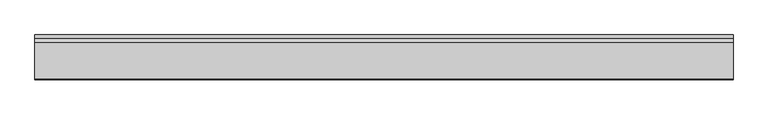
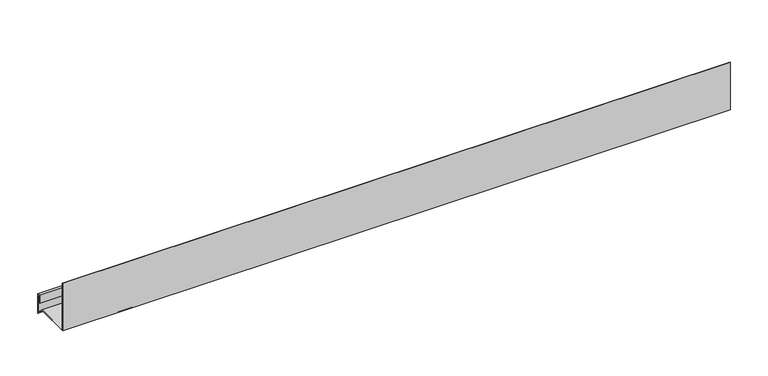
"""IFC4 building model written with IfcOpenShell, lengths in millimetres: proxy geometry, Generic Models 7:Generic Models 1:337419:Generic Models 1:337419 : Generic Models 7:Generic Models 1:337419:2 : Generic Models 7:Generic Models 1:337419:Generic Models 1:337419 : Generic Models 7:Generic Models 1:337419:301336."""

from ifc_helpers import new_model, si_unit, frame, origin, place, context, project, spatial, polyline, outline, extrude, source, transform, mapped, element, save


def generic_models_337c40a0(model_context):
    return source(origin(), model_context, "Body", "SweptSolid", [
        extrude(outline(polyline([(-536494.6078125, 2509.7246799), (-536489.8453125, 2509.7246799), (-536489.8453125, 2477.9746799), (-536501.0706327, 2489.2), (-536554.8784109, 2489.2), (-536554.8784109, 2565.4), (-536554.0846609, 2565.4), (-536554.0846609, 2489.99375), (-536500.7418507, 2489.99375), (-536490.6390625, 2479.8909619), (-536490.6390625, 2508.9309299), (-536493.8140625, 2508.9309299), (-536493.8140625, 2497.0246799), (-536494.6078125, 2497.0246799), (-536494.6078125, 2509.7246799)])), frame((592715.7367242, 0.0, 0.0), z_axis=(1.0, 0.0, 0.0), x_axis=(0.0, 1.0, 0.0)), (0.0, 0.0, 1.0), 1016.0),
    ])


if __name__ == "__main__":
    model = new_model("IFC4")
    model_context = context("Model", 3, world=origin())
    ifc_project = project(units=[si_unit("LENGTHUNIT", "METRE", prefix="MILLI")], contexts=[model_context])
    site = spatial("IfcSite", under=ifc_project)
    building = spatial("IfcBuilding", under=site)
    placement = place(None, origin())
    generic_models_shape = generic_models_337c40a0(model_context)
    element("IfcBuildingElementProxy", 1, Name="Generic Models 7:Generic Models 1:337419:Generic Models 1:337419 : Generic Models 7:Generic Models 1:337419:2 : Generic Models 7:Generic Models 1:337419:Generic Models 1:337419 : Generic Models 7:Generic Models 1:337419:301336", ObjectType="Generic Models 7:Generic Models 1:337419:Generic Models 1:337419 : Generic Models 7:Generic Models 1:337419:2 : Generic Models 7:Generic Models 1:337419:Generic Models 1:337419 : Generic Models 7:Generic Models 1:337419:301336", at=placement, inside=building, context=model_context, shape_type="MappedRepresentation", body=[
        mapped(generic_models_shape, transform((0.0, 0.0, 0.0), x_axis=(1.0, 0.0, 0.0), y_axis=(0.0, 1.0, 0.0), z_axis=(0.0, 0.0, 1.0))),
    ])
    save(model, "model.ifc")

# Revit data of these elements
# Type "Generic Models 7:Generic Models 1:337419:Generic Models 1:337419 : Generic Models 7:Generic Models 1:337419:2 : Generic Models 7:Generic Models 1:337419:Generic Models 1:337419 : Generic Models 7:Generic Models 1:337419:301336"
#   NameOverride = "Generic Models 7:Generic Models 1:337419:Generic Models 1:337419 : Generic Models 7:Generic Models 1:337419:301336"
#   ObjectTypeOverride = "Generic Models 1:337419 : Generic Models 7:Generic Models 1:337419"
#   Reference = "Generic Models 1"
#   Tag = "301336"
# Element 1 (IfcBuildingElementProxy, "Generic Models 7:Generic Models 1:337419:Generic Models 1:337419 : Generic Models 7:Generic Models 1:337419:2 : Generic Models 7:Generic Models 1:337419:Generic Models 1:337419 : Generic Models 7:Generic Models 1:337419:301336")
#   Materials on its faces: "BRAKE METAL FLASHING WITH BACK & END DAMS"
# Materials
#   "BRAKE METAL FLASHING WITH BACK & END DAMS": class "Unassigned", colour RGB 182 182 182, transparency 0, Cost = 0
